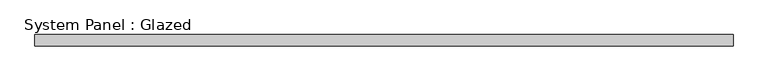
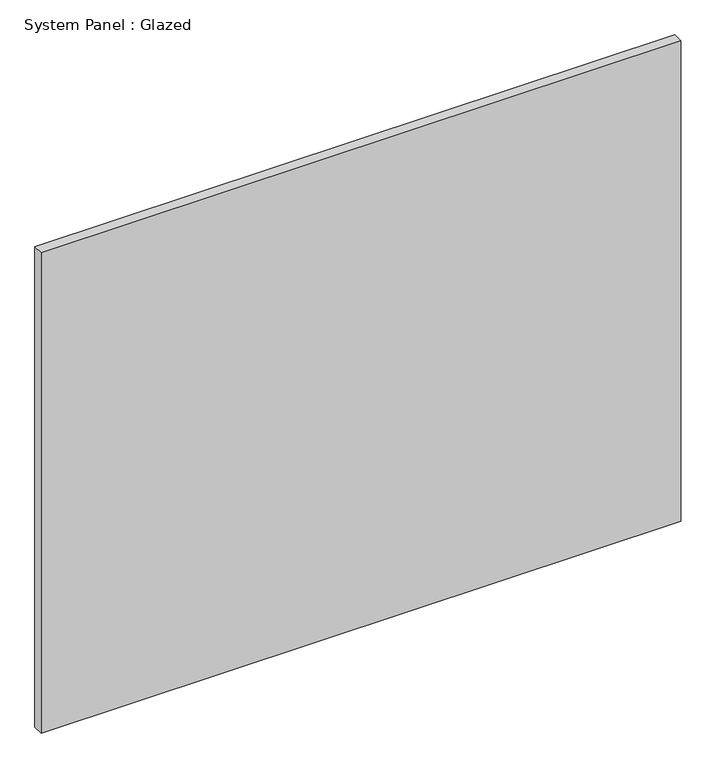
"""IFC4 building model written with IfcOpenShell, lengths in millimetres: plate geometry, System Panel : Glazed."""

import ifcopenshell
import ifcopenshell.guid

model = None  # the IFC model being written
_history = None  # IfcOwnerHistory: only IFC2X3 demands one
_inside = {}  # id of a spatial element -> (the spatial element, [elements in it])
_under = {}  # id of a project, library or spatial element -> (it, [spatial elements below it])
_declared = {}  # id of a project -> (the project, [libraries it declares])
_typed = {}  # id of a type object -> (the type object, [elements of that type])
_made_of = {}  # id of a material, layer set ... -> (it, [elements and type objects made of it])


def new_model(schema):
    """Start an empty IFC model of exactly this schema.

    Asked for "IFC4X3", IfcOpenShell would pick the latest addendum, in which some entities
    have other attributes; the version numbers below select the first issue.
    IFC2X3 requires an IfcOwnerHistory on every rooted entity: one is made here for all.
    """
    global model, _history
    if schema == "IFC4X3":
        model = ifcopenshell.file(schema_version=(4, 3, 0, 0))
    else:
        model = ifcopenshell.file(schema=schema)
    _inside.clear()
    _under.clear()
    _declared.clear()
    _typed.clear()
    _made_of.clear()
    _history = None
    if model.schema == "IFC2X3":
        org = make("IfcOrganization", Name="unknown")
        user = make(
            "IfcPersonAndOrganization",
            ThePerson=make("IfcPerson", FamilyName="unknown"),
            TheOrganization=org,
        )
        app = make(
            "IfcApplication",
            ApplicationDeveloper=org,
            Version="unknown",
            ApplicationFullName="unknown",
            ApplicationIdentifier="unknown",
        )
        _history = make(
            "IfcOwnerHistory",
            OwningUser=user,
            OwningApplication=app,
            ChangeAction="ADDED",
            CreationDate=0,
        )
    return model


def make(cls, **values):
    """One entity of the class cls with the attributes given. An attribute that is None is left unset."""
    return model.create_entity(
        cls, **{name: value for name, value in values.items() if value is not None}
    )


def rooted(cls, **values):
    """An entity with a GlobalId (a new one), such as an element, a storey or a relation."""
    return make(cls, GlobalId=ifcopenshell.guid.new(), OwnerHistory=_history, **values)


def si_unit(unit_type, name, prefix=None):
    """IfcSIUnit, for example si_unit("LENGTHUNIT", "METRE", prefix="MILLI")."""
    return make("IfcSIUnit", UnitType=unit_type, Prefix=prefix, Name=name)


def assignment(units):
    """IfcUnitAssignment: the units of a project."""
    return None if units is None else make("IfcUnitAssignment", Units=units)


def point(xyz):
    """IfcCartesianPoint."""
    return None if xyz is None else make("IfcCartesianPoint", Coordinates=xyz)


def direction(xyz):
    """IfcDirection."""
    return None if xyz is None else make("IfcDirection", DirectionRatios=xyz)


def frame(location, z_axis=None, x_axis=None):
    """IfcAxis2Placement3D, a coordinate frame: its origin and axes. An axis left out is left unset."""
    return make(
        "IfcAxis2Placement3D",
        Location=point(location),
        Axis=direction(z_axis),
        RefDirection=direction(x_axis),
    )


def origin():
    """The frame at (0, 0, 0) with its axes left unset."""
    return frame((0.0, 0.0, 0.0))


def origin_with_axes():
    """The frame at (0, 0, 0) with the z axis (0, 0, 1) and the x axis (1, 0, 0) written out."""
    return frame((0.0, 0.0, 0.0), z_axis=(0.0, 0.0, 1.0), x_axis=(1.0, 0.0, 0.0))


def place(relative_to, where):
    """IfcLocalPlacement: puts the frame where relative to a parent placement (None: the world)."""
    return make(
        "IfcLocalPlacement", PlacementRelTo=relative_to, RelativePlacement=where
    )


def context(
    kind, dimensions, precision=None, world=None, true_north=None, identifier=None
):
    """IfcGeometricRepresentationContext, for example the 3D "Model" context."""
    return make(
        "IfcGeometricRepresentationContext",
        ContextIdentifier=identifier,
        ContextType=kind,
        CoordinateSpaceDimension=dimensions,
        Precision=precision,
        WorldCoordinateSystem=world,
        TrueNorth=true_north,
    )


def project(units=None, contexts=None):
    """IfcProject with its units and contexts."""
    return rooted(
        "IfcProject",
        Name="project",
        RepresentationContexts=contexts,
        UnitsInContext=assignment(units),
    )


def spatial(cls, under=None, at=None, **own):
    """A site, building, storey or space (cls), placed at a placement, below another one or the project."""
    s = rooted(cls, ObjectPlacement=at, **own)
    if under is not None:
        _under.setdefault(under.id(), (under, []))[1].append(s)
    return s


def polyline(points):
    """IfcPolyline through the points."""
    return make("IfcPolyline", Points=[point(p) for p in points])


def outline(outer, holes=None, kind="AREA"):
    """IfcArbitraryClosedProfileDef: a profile drawn as a closed curve; with holes, ...WithVoids."""
    if holes is None:
        return make("IfcArbitraryClosedProfileDef", ProfileType=kind, OuterCurve=outer)
    return make(
        "IfcArbitraryProfileDefWithVoids",
        ProfileType=kind,
        OuterCurve=outer,
        InnerCurves=holes,
    )


def extrude(swept, where, along, depth):
    """IfcExtrudedAreaSolid: the profile swept, set in the frame where, extruded along a direction by depth."""
    return make(
        "IfcExtrudedAreaSolid",
        SweptArea=swept,
        Position=where,
        ExtrudedDirection=direction(along),
        Depth=depth,
    )


def shape(context_of_items, identifier, shape_type, items):
    """IfcShapeRepresentation: the items that make up one representation, for example the "Body"."""
    return make(
        "IfcShapeRepresentation",
        ContextOfItems=context_of_items,
        RepresentationIdentifier=identifier,
        RepresentationType=shape_type,
        Items=items,
    )


def source(mapping_origin, context_of_items, identifier, shape_type, items):
    """IfcRepresentationMap: a shape defined once, which mapped items show again and again."""
    return make(
        "IfcRepresentationMap",
        MappingOrigin=mapping_origin,
        MappedRepresentation=shape(context_of_items, identifier, shape_type, items),
    )


def transform(
    local_origin,
    x_axis=None,
    y_axis=None,
    z_axis=None,
    scale=None,
    scale2=None,
    scale3=None,
    uniform=True,
):
    """IfcCartesianTransformationOperator3D, or its non-uniform kind. x_axis, y_axis, z_axis: its Axis1, 2, 3."""
    if uniform:
        return make(
            "IfcCartesianTransformationOperator3D",
            Axis1=direction(x_axis),
            Axis2=direction(y_axis),
            LocalOrigin=point(local_origin),
            Scale=scale,
            Axis3=direction(z_axis),
        )
    return make(
        "IfcCartesianTransformationOperator3DnonUniform",
        Axis1=direction(x_axis),
        Axis2=direction(y_axis),
        LocalOrigin=point(local_origin),
        Scale=scale,
        Axis3=direction(z_axis),
        Scale2=scale2,
        Scale3=scale3,
    )


def mapped(mapping_source, mapping_target):
    """IfcMappedItem: shows the shape of a source again, moved by a transform."""
    return make(
        "IfcMappedItem", MappingSource=mapping_source, MappingTarget=mapping_target
    )


def made_of(thing, what):
    """Note that an element or type object is made of a material, layer set ...; save() writes the relation."""
    if what is not None:
        _made_of.setdefault(what.id(), (what, []))[1].append(thing)
    return thing


def element(
    cls,
    number,
    at=None,
    inside=None,
    cuts=None,
    type_object=None,
    material=None,
    context=None,
    identifier="Body",
    shape_type=None,
    held_by="IfcProductDefinitionShape",
    body=None,
    shapes=None,
    **own,
):
    """One element of the class cls, such as IfcWall. Its Tag is "e" and its number.

    at: its placement. inside: the storey or other place that contains it. cuts: it is an
    opening in that element (IfcRelVoidsElement). A single representation is given by context,
    identifier, shape_type and body (its items); several are given by shapes. held_by: the class
    of the entity that holds the representations. save() writes the other relations.
    """
    e = rooted(cls, Tag="e%d" % number, ObjectPlacement=at, **own)
    if body is not None:
        shapes = [shape(context, identifier, shape_type, body)]
    if shapes is not None:
        e.Representation = make(held_by, Representations=shapes)
    if inside is not None:
        _inside.setdefault(inside.id(), (inside, []))[1].append(e)
    if cuts is not None:
        rooted(
            "IfcRelVoidsElement", RelatingBuildingElement=cuts, RelatedOpeningElement=e
        )
    if type_object is not None:
        _typed.setdefault(type_object.id(), (type_object, []))[1].append(e)
    return made_of(e, material)


def aggregate(whole, parts):
    """IfcRelAggregates: a whole, such as a stair, and the parts it consists of."""
    return rooted("IfcRelAggregates", RelatingObject=whole, RelatedObjects=parts)


def save(model, path):
    """Write the relations noted so far, then the file.

    IfcRelAggregates (storeys below a building ...), IfcRelContainedInSpatialStructure (elements
    in a storey), IfcRelDefinesByType, IfcRelAssociatesMaterial and IfcRelDeclares: one each for
    every whole, place, type object, material and project.
    """
    for whole, parts in _under.values():
        aggregate(whole, parts)
    for where, things in _inside.values():
        rooted(
            "IfcRelContainedInSpatialStructure",
            RelatedElements=things,
            RelatingStructure=where,
        )
    for kind, things in _typed.values():
        rooted("IfcRelDefinesByType", RelatedObjects=things, RelatingType=kind)
    for what, things in _made_of.values():
        rooted("IfcRelAssociatesMaterial", RelatedObjects=things, RelatingMaterial=what)
    for by, libraries in _declared.values():
        rooted("IfcRelDeclares", RelatingContext=by, RelatedDefinitions=libraries)
    model.write(path)


def system_panel_glazed_4ad6d596(model_context):
    return source(origin(), model_context, "Body", "SweptSolid", [
        extrude(outline(polyline([(768.35, 19.05), (-768.35, 19.05), (-768.35, 44.45), (768.35, 44.45), (768.35, 19.05)])), origin_with_axes(), (0.0, 0.0, 1.0), 1219.2),
    ])


if __name__ == "__main__":
    model = new_model("IFC4")
    model_context = context("Model", 3, world=origin())
    ifc_project = project(units=[si_unit("LENGTHUNIT", "METRE", prefix="MILLI")], contexts=[model_context])
    site = spatial("IfcSite", under=ifc_project)
    building = spatial("IfcBuilding", under=site)
    placement = place(None, origin())
    system_panel_glazed_shape = system_panel_glazed_4ad6d596(model_context)
    element("IfcPlate", 1, ObjectType="System Panel : Glazed", at=placement, inside=building, context=model_context, shape_type="MappedRepresentation", body=[
        mapped(system_panel_glazed_shape, transform((0.0, 0.0, 0.0), x_axis=(1.0, 0.0, 0.0), y_axis=(0.0, 1.0, 0.0), z_axis=(0.0, 0.0, 1.0))),
    ])
    save(model, "model.ifc")

# Revit data of these elements
# Element 1 (IfcPlate, "System Panel : Glazed")
#   Materials on its faces: "Glass"
# Materials
#   "Glass": class "Glass", colour RGB 0 128 192, transparency 0.75
